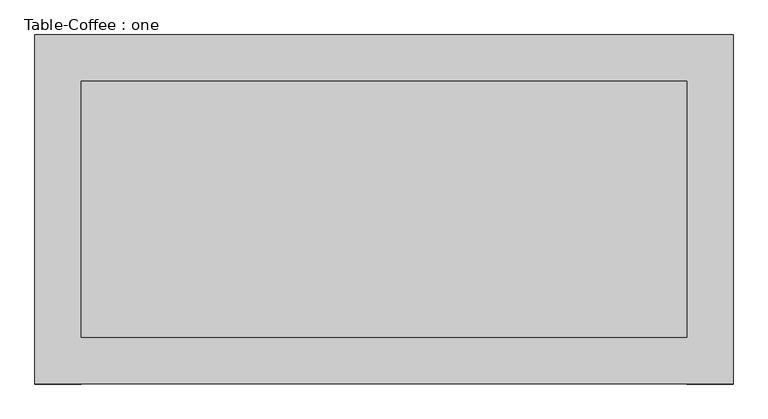
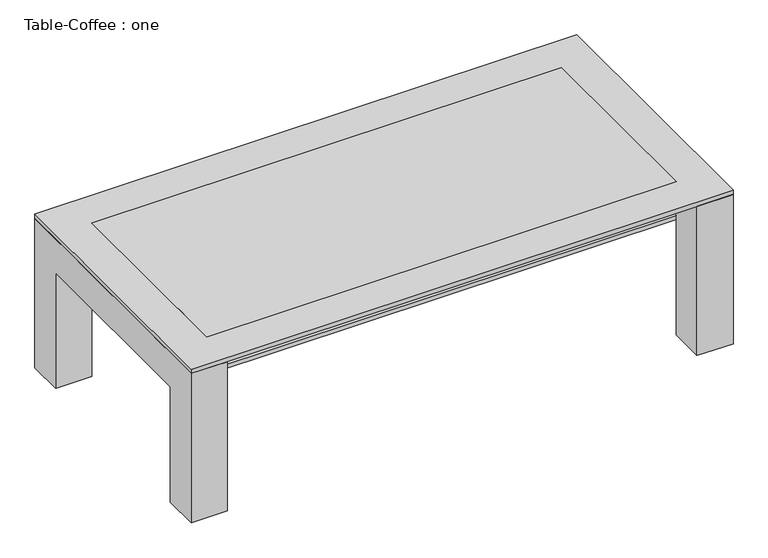
"""IFC4 building model written with IfcOpenShell, lengths in millimetres: furniture geometry, Table-Coffee : one."""

from ifc_helpers import new_model, si_unit, frame, origin, place, context, project, spatial, polyline, outline, extrude, source, transform, mapped, element, save


def table_coffee_one_162ba504(model_context):
    return source(origin(), model_context, "Body", "SweptSolid", [
        extrude(outline(polyline([(678.6657667, 374.6110778), (678.6657667, -184.1889222), (-642.1342333, -184.1889222), (-642.1342333, 374.6110778), (678.6657667, 374.6110778)])), frame((0.0, 0.0, 342.9), z_axis=(0.0, 0.0, 1.0), x_axis=(1.0, 0.0, 0.0)), (0.0, 0.0, 1.0), 12.7),
        extrude(outline(polyline([(476.2110778, 0.0), (374.6110778, 0.0), (374.6110778, 342.9), (-184.1889222, 342.9), (-184.1889222, 0.0), (-285.7889222, 0.0), (-285.7889222, 444.5), (476.2110778, 444.5), (476.2110778, 0.0)])), frame((678.6657667, 0.0, 0.0), z_axis=(1.0, 0.0, 0.0), x_axis=(0.0, 1.0, 0.0)), (0.0, 0.0, 1.0), 101.6),
        extrude(outline(polyline([(476.2110778, 444.5), (476.2110778, 0.0), (374.6110778, 0.0), (374.6110778, 342.9), (-184.1889222, 342.9), (-184.1889222, 0.0), (-285.7889222, 0.0), (-285.7889222, 444.5), (476.2110778, 444.5)])), frame((-743.7342333, 0.0, 0.0), z_axis=(1.0, 0.0, 0.0), x_axis=(0.0, 1.0, 0.0)), (0.0, 0.0, 1.0), 101.6),
        extrude(outline(polyline([(678.6657667, 374.6110778), (678.6657667, -184.1889222), (-642.1342333, -184.1889222), (-642.1342333, 374.6110778), (678.6657667, 374.6110778)])), frame((0.0, 0.0, 444.5), z_axis=(0.0, 0.0, 1.0), x_axis=(1.0, 0.0, 0.0)), (0.0, 0.0, 1.0), 12.7),
        extrude(outline(polyline([(780.2657667, 476.2110778), (780.2657667, -285.7889222), (-743.7342333, -285.7889222), (-743.7342333, 476.2110778), (780.2657667, 476.2110778)]), holes=[polyline([(678.6657667, 374.6110778), (-642.1342333, 374.6110778), (-642.1342333, -184.1889222), (678.6657667, -184.1889222), (678.6657667, 374.6110778)])]), frame((0.0, 0.0, 444.5), z_axis=(0.0, 0.0, 1.0), x_axis=(1.0, 0.0, 0.0)), (0.0, 0.0, 1.0), 12.7),
    ])


if __name__ == "__main__":
    model = new_model("IFC4")
    model_context = context("Model", 3, world=origin())
    ifc_project = project(units=[si_unit("LENGTHUNIT", "METRE", prefix="MILLI")], contexts=[model_context])
    site = spatial("IfcSite", under=ifc_project)
    building = spatial("IfcBuilding", under=site)
    placement = place(None, origin())
    table_coffee_one_shape = table_coffee_one_162ba504(model_context)
    element("IfcFurniture", 1, ObjectType="Table-Coffee : one", at=placement, inside=building, context=model_context, shape_type="MappedRepresentation", body=[
        mapped(table_coffee_one_shape, transform((0.0, 0.0, 0.0), x_axis=(1.0, 0.0, 0.0), y_axis=(0.0, 1.0, 0.0), z_axis=(0.0, 0.0, 1.0))),
    ])
    save(model, "model.ifc")

# Revit data of these elements
# Type "Table-Coffee : one"
#   Assembly Code = "E2020200"
#   Height = 1' - 6"
#   Length = 5' - 0"
#   Width = 2' - 6"
#   Top Material = Metal - Chrome
#   Frame Material = Wood - Teak
# Element 1 (IfcFurniture, "Table-Coffee : one")
#   Materials on its faces: "Wood - Teak", "Metal - Chrome", "Glass - Clear, Grey"
# Materials
#   "Metal - Chrome": class "Metal", colour RGB 17 17 17, transparency 0
#   "Wood - Teak": class "Wood", colour RGB 145 112 90, transparency 0
#   "Glass - Clear, Grey": class "Glass", colour RGB 252 255 255, transparency 0.64
